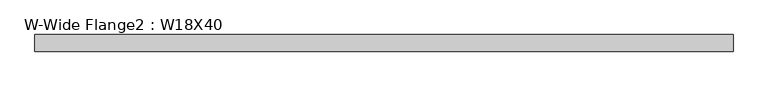
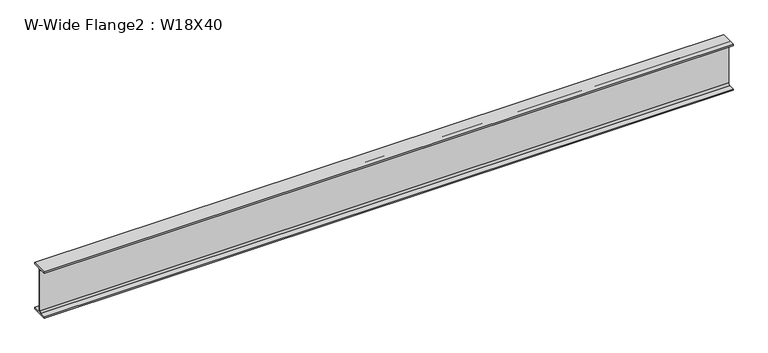
"""IFC4 building model written with IfcOpenShell, lengths in millimetres: beam geometry, W-Wide Flange2 : W18X40."""

from ifc_helpers import new_model, si_unit, point, frame, frame_2d, origin, place, context, project, spatial, polyline, circle_curve, trimmed, segment, composite_curve, outline, extrude, source, transform, mapped, element, save


def w_wide_flange2_w18x40_cea889e1(model_context):
    return source(origin(), model_context, "Body", "SweptSolid", [
        extrude(outline(composite_curve([segment(polyline([(76.454, -213.995), (76.454, -227.33), (-76.454, -227.33), (-76.454, -213.995), (-20.828, -213.995)]), True, "CONTINUOUS"), segment(trimmed(circle_curve(frame_2d((-20.828, -197.1675)), 16.8275), [point((-20.828, -213.995))], [point((-4.0005, -197.1675))], True, "CARTESIAN"), True, "CONTINUOUS"), segment(polyline([(-4.0005, -197.1675), (-4.0005, 197.1675)]), True, "CONTINUOUS"), segment(trimmed(circle_curve(frame_2d((-20.828, 197.1675)), 16.8275), [point((-4.0005, 197.1675))], [point((-20.828, 213.995))], True, "CARTESIAN"), True, "CONTINUOUS"), segment(polyline([(-20.828, 213.995), (-76.454, 213.995), (-76.454, 227.33), (76.454, 227.33), (76.454, 213.995), (20.828, 213.995)]), True, "CONTINUOUS"), segment(trimmed(circle_curve(frame_2d((20.828, 197.1675)), 16.8275), [point((20.828, 213.995))], [point((4.0005, 197.1675))], True, "CARTESIAN"), True, "CONTINUOUS"), segment(polyline([(4.0005, 197.1675), (4.0005, -197.1675)]), True, "CONTINUOUS"), segment(trimmed(circle_curve(frame_2d((20.828, -197.1675)), 16.8275), [point((4.0005, -197.1675))], [point((20.828, -213.995))], True, "CARTESIAN"), True, "CONTINUOUS"), segment(polyline([(20.828, -213.995), (76.454, -213.995)]), True, "CONTINUOUS")], self_intersect=False)), frame((-3211.5125, 0.0, 0.0), z_axis=(1.0, 0.0, 0.0), x_axis=(0.0, 1.0, 0.0)), (0.0, 0.0, 1.0), 6417.865625),
    ])


if __name__ == "__main__":
    model = new_model("IFC4")
    model_context = context("Model", 3, world=origin())
    ifc_project = project(units=[si_unit("LENGTHUNIT", "METRE", prefix="MILLI")], contexts=[model_context])
    site = spatial("IfcSite", under=ifc_project)
    building = spatial("IfcBuilding", under=site)
    placement = place(None, origin())
    w_wide_flange2_w18x40_shape = w_wide_flange2_w18x40_cea889e1(model_context)
    element("IfcBeam", 1, ObjectType="W-Wide Flange2 : W18X40", at=placement, inside=building, context=model_context, shape_type="MappedRepresentation", body=[
        mapped(w_wide_flange2_w18x40_shape, transform((0.0, 0.0, 0.0), x_axis=(1.0, 0.0, 0.0), y_axis=(0.0, 1.0, 0.0), z_axis=(0.0, 0.0, 1.0))),
    ])
    save(model, "model.ifc")

# Revit data of these elements
# Type "W-Wide Flange2 : W18X40"
#   Assembly Code = "B10"
#   W = 40
#   Length [instance default] = 5' - 0"
#   bf = 0' - 6.02"
#   d = 1' - 5.9"
#   k = 0' - 1 3/16"
#   k2 = 0' - 0.6625"
#   tf = 0' - 0.525"
#   tw = 0' - 0.315"
#   A = 0.0819444 SF
#   Structural Material [instance default] = Steel ASTM A992
# Element 1 (IfcBeam, "W-Wide Flange2 : W18X40")
#   Materials on its faces: "Steel ASTM A992"
# Materials
#   "Steel ASTM A992": class "Metal", colour RGB 199 199 199, transparency 0, Description = "Structural steel 50ksi", Cost = 0
